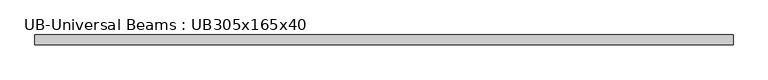
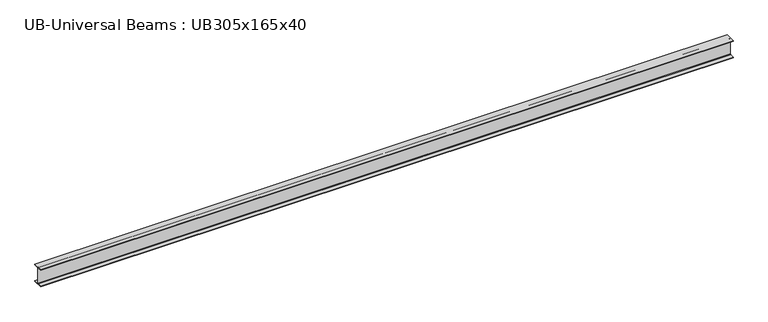
"""IFC4 building model written with IfcOpenShell, lengths in millimetres: member geometry, UB-Universal Beams : UB305x165x40."""

from ifc_helpers import new_model, si_unit, point, frame, frame_2d, origin, place, context, project, spatial, polyline, circle_curve, trimmed, segment, composite_curve, outline, extrude, source, transform, mapped, element, save


def ub_universal_beams_ub305x165x40_793367f0(model_context):
    return source(origin(), model_context, "Body", "SweptSolid", [
        extrude(outline(composite_curve([segment(polyline([(82.5, -141.5), (82.5, -151.7), (-82.5, -151.7), (-82.5, -141.5), (-11.9, -141.5)]), True, "CONTINUOUS"), segment(trimmed(circle_curve(frame_2d((-11.9, -132.6)), 8.9), [point((-11.9, -141.5))], [point((-3.0, -132.6))], True, "CARTESIAN"), True, "CONTINUOUS"), segment(polyline([(-3.0, -132.6), (-3.0, 132.6)]), True, "CONTINUOUS"), segment(trimmed(circle_curve(frame_2d((-11.9, 132.6)), 8.9), [point((-3.0, 132.6))], [point((-11.9, 141.5))], True, "CARTESIAN"), True, "CONTINUOUS"), segment(polyline([(-11.9, 141.5), (-82.5, 141.5), (-82.5, 151.7), (82.5, 151.7), (82.5, 141.5), (11.9, 141.5)]), True, "CONTINUOUS"), segment(trimmed(circle_curve(frame_2d((11.9, 132.6)), 8.9), [point((11.9, 141.5))], [point((3.0, 132.6))], True, "CARTESIAN"), True, "CONTINUOUS"), segment(polyline([(3.0, 132.6), (3.0, -132.6)]), True, "CONTINUOUS"), segment(trimmed(circle_curve(frame_2d((11.9, -132.6)), 8.9), [point((3.0, -132.6))], [point((11.9, -141.5))], True, "CARTESIAN"), True, "CONTINUOUS"), segment(polyline([(11.9, -141.5), (82.5, -141.5)]), True, "CONTINUOUS")], self_intersect=False)), frame((-5600.7, 0.0, 0.0), z_axis=(1.0, 0.0, 0.0), x_axis=(0.0, 1.0, 0.0)), (0.0, 0.0, 1.0), 11654.3),
    ])


if __name__ == "__main__":
    model = new_model("IFC4")
    model_context = context("Model", 3, world=origin())
    ifc_project = project(units=[si_unit("LENGTHUNIT", "METRE", prefix="MILLI")], contexts=[model_context])
    site = spatial("IfcSite", under=ifc_project)
    building = spatial("IfcBuilding", under=site)
    placement = place(None, origin())
    ub_universal_beams_ub305x165x40_shape = ub_universal_beams_ub305x165x40_793367f0(model_context)
    element("IfcMember", 1, ObjectType="UB-Universal Beams : UB305x165x40", at=placement, inside=building, context=model_context, shape_type="MappedRepresentation", body=[
        mapped(ub_universal_beams_ub305x165x40_shape, transform((0.0, 0.0, 0.0), x_axis=(1.0, 0.0, 0.0), y_axis=(0.0, 1.0, 0.0), z_axis=(0.0, 0.0, 1.0))),
    ])
    save(model, "model.ifc")

# Revit data of these elements
# Type "UB-Universal Beams : UB305x165x40"
#   Section Name Key = "UB305X165X40"
#   Width = 16.5 cm
#   Web Thickness = 0.6 cm
#   Web Fillet = 0.89 cm
#   Warping Constant = 164000.0 cm⁶
#   Torsional Moment of Inertia = 14.70 cm⁴
#   Section Area = 51.3 cm²
#   Plastic Modulus weak axis = 142.0 cm³
#   Plastic Modulus strong axis = 623.0 cm³
#   Nominal Weight = 40.2999 kgf/m
#   Moment of Inertia weak axis = 764.00 cm⁴
#   Moment of Inertia strong axis = 8503.00 cm⁴
#   Height = 30.34 cm
#   Flange Thickness = 1.02 cm
#   Elastic Modulus weak axis = 92.6 cm³
#   Elastic Modulus strong axis = 560.0 cm³
#   Centroid Vertical = 15.17 cm
#   Centroid Horizontal = 8.25 cm
#   Bolt Spacing = 9.0 cm
#   Length [instance default] = 1500 mm
#   Structural Material [instance default] = Metal - Steel 43-275
#   Type Comments = ""
#   Assembly Code = ""
# Element 1 (IfcMember, "UB-Universal Beams : UB305x165x40")
#   Materials on its faces: "Metal - Steel 43-275"
# Materials
#   "Metal - Steel 43-275": class "Metal", colour RGB 247 247 247, transparency 0, Cost = 0
